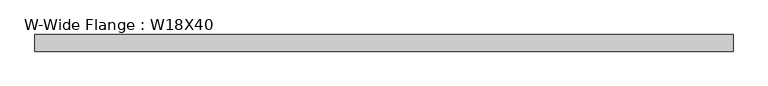
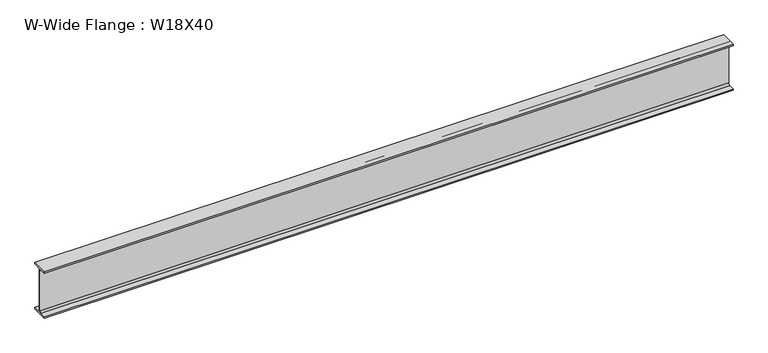
"""IFC4 building model written with IfcOpenShell, lengths in millimetres: beam geometry, W-Wide Flange : W18X40."""

from ifc_helpers import new_model, si_unit, point, frame, frame_2d, origin, place, context, project, spatial, polyline, circle_curve, trimmed, segment, composite_curve, outline, extrude, source, transform, mapped, element, save


def w_wide_flange_w18x40_26c92dcf(model_context):
    return source(origin(), model_context, "Body", "SweptSolid", [
        extrude(outline(composite_curve([segment(polyline([(76.454, -213.995), (76.454, -227.33), (-76.454, -227.33), (-76.454, -213.995), (-20.828, -213.995)]), True, "CONTINUOUS"), segment(trimmed(circle_curve(frame_2d((-20.828, -197.1675)), 16.8275), [point((-20.828, -213.995))], [point((-4.0005, -197.1675))], True, "CARTESIAN"), True, "CONTINUOUS"), segment(polyline([(-4.0005, -197.1675), (-4.0005, 197.1675)]), True, "CONTINUOUS"), segment(trimmed(circle_curve(frame_2d((-20.828, 197.1675)), 16.8275), [point((-4.0005, 197.1675))], [point((-20.828, 213.995))], True, "CARTESIAN"), True, "CONTINUOUS"), segment(polyline([(-20.828, 213.995), (-76.454, 213.995), (-76.454, 227.33), (76.454, 227.33), (76.454, 213.995), (20.828, 213.995)]), True, "CONTINUOUS"), segment(trimmed(circle_curve(frame_2d((20.828, 197.1675)), 16.8275), [point((20.828, 213.995))], [point((4.0005, 197.1675))], True, "CARTESIAN"), True, "CONTINUOUS"), segment(polyline([(4.0005, 197.1675), (4.0005, -197.1675)]), True, "CONTINUOUS"), segment(trimmed(circle_curve(frame_2d((20.828, -197.1675)), 16.8275), [point((4.0005, -197.1675))], [point((20.828, -213.995))], True, "CARTESIAN"), True, "CONTINUOUS"), segment(polyline([(20.828, -213.995), (76.454, -213.995)]), True, "CONTINUOUS")], self_intersect=False)), frame((-3211.83, 0.0, 0.0), z_axis=(1.0, 0.0, 0.0), x_axis=(0.0, 1.0, 0.0)), (0.0, 0.0, 1.0), 6418.58),
    ])


if __name__ == "__main__":
    model = new_model("IFC4")
    model_context = context("Model", 3, world=origin())
    ifc_project = project(units=[si_unit("LENGTHUNIT", "METRE", prefix="MILLI")], contexts=[model_context])
    site = spatial("IfcSite", under=ifc_project)
    building = spatial("IfcBuilding", under=site)
    placement = place(None, origin())
    w_wide_flange_w18x40_shape = w_wide_flange_w18x40_26c92dcf(model_context)
    element("IfcBeam", 1, ObjectType="W-Wide Flange : W18X40", at=placement, inside=building, context=model_context, shape_type="MappedRepresentation", body=[
        mapped(w_wide_flange_w18x40_shape, transform((0.0, 0.0, 0.0), x_axis=(1.0, 0.0, 0.0), y_axis=(0.0, 1.0, 0.0), z_axis=(0.0, 0.0, 1.0))),
    ])
    save(model, "model.ifc")

# Revit data of these elements
# Type "W-Wide Flange : W18X40"
#   Assembly Code = "B10"
#   W = 40
#   Length [instance default] = 5' - 0"
#   bf = 0' - 6.02"
#   d = 1' - 5.9"
#   k = 0' - 1 3/16"
#   k2 = 0' - 0.6625"
#   tf = 0' - 0.525"
#   tw = 0' - 0.315"
#   A = 0.0819444 SF
#   Structural Material [instance default] = Steel ASTM A992
# Element 1 (IfcBeam, "W-Wide Flange : W18X40")
#   Materials on its faces: "Steel ASTM A992"
# Materials
#   "Steel ASTM A992": class "Metal", colour RGB 199 199 199, transparency 0, Description = "Structural steel 50ksi", Cost = 0
